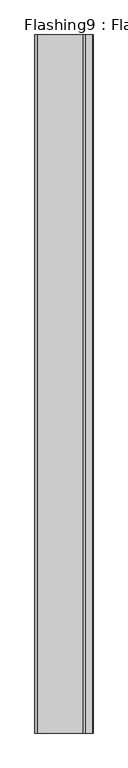
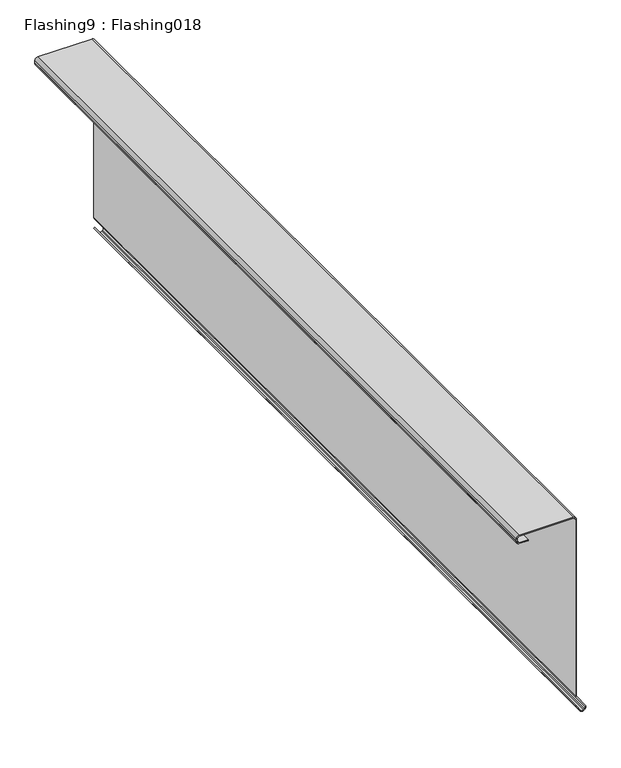
"""IFC4 building model written with IfcOpenShell, lengths in millimetres: proxy geometry, Flashing9 : Flashing018."""

import ifcopenshell
import ifcopenshell.guid

model = None  # the IFC model being written
_history = None  # IfcOwnerHistory: only IFC2X3 demands one
_inside = {}  # id of a spatial element -> (the spatial element, [elements in it])
_under = {}  # id of a project, library or spatial element -> (it, [spatial elements below it])
_declared = {}  # id of a project -> (the project, [libraries it declares])
_typed = {}  # id of a type object -> (the type object, [elements of that type])
_made_of = {}  # id of a material, layer set ... -> (it, [elements and type objects made of it])


def new_model(schema):
    """Start an empty IFC model of exactly this schema.

    Asked for "IFC4X3", IfcOpenShell would pick the latest addendum, in which some entities
    have other attributes; the version numbers below select the first issue.
    IFC2X3 requires an IfcOwnerHistory on every rooted entity: one is made here for all.
    """
    global model, _history
    if schema == "IFC4X3":
        model = ifcopenshell.file(schema_version=(4, 3, 0, 0))
    else:
        model = ifcopenshell.file(schema=schema)
    _inside.clear()
    _under.clear()
    _declared.clear()
    _typed.clear()
    _made_of.clear()
    _history = None
    if model.schema == "IFC2X3":
        org = make("IfcOrganization", Name="unknown")
        user = make(
            "IfcPersonAndOrganization",
            ThePerson=make("IfcPerson", FamilyName="unknown"),
            TheOrganization=org,
        )
        app = make(
            "IfcApplication",
            ApplicationDeveloper=org,
            Version="unknown",
            ApplicationFullName="unknown",
            ApplicationIdentifier="unknown",
        )
        _history = make(
            "IfcOwnerHistory",
            OwningUser=user,
            OwningApplication=app,
            ChangeAction="ADDED",
            CreationDate=0,
        )
    return model


def make(cls, **values):
    """One entity of the class cls with the attributes given. An attribute that is None is left unset."""
    return model.create_entity(
        cls, **{name: value for name, value in values.items() if value is not None}
    )


def rooted(cls, **values):
    """An entity with a GlobalId (a new one), such as an element, a storey or a relation."""
    return make(cls, GlobalId=ifcopenshell.guid.new(), OwnerHistory=_history, **values)


def si_unit(unit_type, name, prefix=None):
    """IfcSIUnit, for example si_unit("LENGTHUNIT", "METRE", prefix="MILLI")."""
    return make("IfcSIUnit", UnitType=unit_type, Prefix=prefix, Name=name)


def assignment(units):
    """IfcUnitAssignment: the units of a project."""
    return None if units is None else make("IfcUnitAssignment", Units=units)


def point(xyz):
    """IfcCartesianPoint."""
    return None if xyz is None else make("IfcCartesianPoint", Coordinates=xyz)


def direction(xyz):
    """IfcDirection."""
    return None if xyz is None else make("IfcDirection", DirectionRatios=xyz)


def frame(location, z_axis=None, x_axis=None):
    """IfcAxis2Placement3D, a coordinate frame: its origin and axes. An axis left out is left unset."""
    return make(
        "IfcAxis2Placement3D",
        Location=point(location),
        Axis=direction(z_axis),
        RefDirection=direction(x_axis),
    )


def frame_2d(location, x_axis=None):
    """IfcAxis2Placement2D, a coordinate frame in the plane: its origin and x axis."""
    return make(
        "IfcAxis2Placement2D", Location=point(location), RefDirection=direction(x_axis)
    )


def origin():
    """The frame at (0, 0, 0) with its axes left unset."""
    return frame((0.0, 0.0, 0.0))


def place(relative_to, where):
    """IfcLocalPlacement: puts the frame where relative to a parent placement (None: the world)."""
    return make(
        "IfcLocalPlacement", PlacementRelTo=relative_to, RelativePlacement=where
    )


def context(
    kind, dimensions, precision=None, world=None, true_north=None, identifier=None
):
    """IfcGeometricRepresentationContext, for example the 3D "Model" context."""
    return make(
        "IfcGeometricRepresentationContext",
        ContextIdentifier=identifier,
        ContextType=kind,
        CoordinateSpaceDimension=dimensions,
        Precision=precision,
        WorldCoordinateSystem=world,
        TrueNorth=true_north,
    )


def project(units=None, contexts=None):
    """IfcProject with its units and contexts."""
    return rooted(
        "IfcProject",
        Name="project",
        RepresentationContexts=contexts,
        UnitsInContext=assignment(units),
    )


def spatial(cls, under=None, at=None, **own):
    """A site, building, storey or space (cls), placed at a placement, below another one or the project."""
    s = rooted(cls, ObjectPlacement=at, **own)
    if under is not None:
        _under.setdefault(under.id(), (under, []))[1].append(s)
    return s


def polyline(points):
    """IfcPolyline through the points."""
    return make("IfcPolyline", Points=[point(p) for p in points])


def circle_curve(where, radius):
    """IfcCircle in the frame where."""
    return make("IfcCircle", Position=where, Radius=radius)


def trimmed(basis, trim1, trim2, sense, master):
    """IfcTrimmedCurve: the piece of a basis curve between two trims."""
    return make(
        "IfcTrimmedCurve",
        BasisCurve=basis,
        Trim1=trim1,
        Trim2=trim2,
        SenseAgreement=sense,
        MasterRepresentation=master,
    )


def segment(curve, same_sense, transition):
    """IfcCompositeCurveSegment."""
    return make(
        "IfcCompositeCurveSegment",
        Transition=transition,
        SameSense=same_sense,
        ParentCurve=curve,
    )


def composite_curve(segments, self_intersect=None):
    """IfcCompositeCurve: segments joined end to end."""
    return make("IfcCompositeCurve", Segments=segments, SelfIntersect=self_intersect)


def outline(outer, holes=None, kind="AREA"):
    """IfcArbitraryClosedProfileDef: a profile drawn as a closed curve; with holes, ...WithVoids."""
    if holes is None:
        return make("IfcArbitraryClosedProfileDef", ProfileType=kind, OuterCurve=outer)
    return make(
        "IfcArbitraryProfileDefWithVoids",
        ProfileType=kind,
        OuterCurve=outer,
        InnerCurves=holes,
    )


def extrude(swept, where, along, depth):
    """IfcExtrudedAreaSolid: the profile swept, set in the frame where, extruded along a direction by depth."""
    return make(
        "IfcExtrudedAreaSolid",
        SweptArea=swept,
        Position=where,
        ExtrudedDirection=direction(along),
        Depth=depth,
    )


def shape(context_of_items, identifier, shape_type, items):
    """IfcShapeRepresentation: the items that make up one representation, for example the "Body"."""
    return make(
        "IfcShapeRepresentation",
        ContextOfItems=context_of_items,
        RepresentationIdentifier=identifier,
        RepresentationType=shape_type,
        Items=items,
    )


def source(mapping_origin, context_of_items, identifier, shape_type, items):
    """IfcRepresentationMap: a shape defined once, which mapped items show again and again."""
    return make(
        "IfcRepresentationMap",
        MappingOrigin=mapping_origin,
        MappedRepresentation=shape(context_of_items, identifier, shape_type, items),
    )


def transform(
    local_origin,
    x_axis=None,
    y_axis=None,
    z_axis=None,
    scale=None,
    scale2=None,
    scale3=None,
    uniform=True,
):
    """IfcCartesianTransformationOperator3D, or its non-uniform kind. x_axis, y_axis, z_axis: its Axis1, 2, 3."""
    if uniform:
        return make(
            "IfcCartesianTransformationOperator3D",
            Axis1=direction(x_axis),
            Axis2=direction(y_axis),
            LocalOrigin=point(local_origin),
            Scale=scale,
            Axis3=direction(z_axis),
        )
    return make(
        "IfcCartesianTransformationOperator3DnonUniform",
        Axis1=direction(x_axis),
        Axis2=direction(y_axis),
        LocalOrigin=point(local_origin),
        Scale=scale,
        Axis3=direction(z_axis),
        Scale2=scale2,
        Scale3=scale3,
    )


def mapped(mapping_source, mapping_target):
    """IfcMappedItem: shows the shape of a source again, moved by a transform."""
    return make(
        "IfcMappedItem", MappingSource=mapping_source, MappingTarget=mapping_target
    )


def made_of(thing, what):
    """Note that an element or type object is made of a material, layer set ...; save() writes the relation."""
    if what is not None:
        _made_of.setdefault(what.id(), (what, []))[1].append(thing)
    return thing


def element(
    cls,
    number,
    at=None,
    inside=None,
    cuts=None,
    type_object=None,
    material=None,
    context=None,
    identifier="Body",
    shape_type=None,
    held_by="IfcProductDefinitionShape",
    body=None,
    shapes=None,
    **own,
):
    """One element of the class cls, such as IfcWall. Its Tag is "e" and its number.

    at: its placement. inside: the storey or other place that contains it. cuts: it is an
    opening in that element (IfcRelVoidsElement). A single representation is given by context,
    identifier, shape_type and body (its items); several are given by shapes. held_by: the class
    of the entity that holds the representations. save() writes the other relations.
    """
    e = rooted(cls, Tag="e%d" % number, ObjectPlacement=at, **own)
    if body is not None:
        shapes = [shape(context, identifier, shape_type, body)]
    if shapes is not None:
        e.Representation = make(held_by, Representations=shapes)
    if inside is not None:
        _inside.setdefault(inside.id(), (inside, []))[1].append(e)
    if cuts is not None:
        rooted(
            "IfcRelVoidsElement", RelatingBuildingElement=cuts, RelatedOpeningElement=e
        )
    if type_object is not None:
        _typed.setdefault(type_object.id(), (type_object, []))[1].append(e)
    return made_of(e, material)


def aggregate(whole, parts):
    """IfcRelAggregates: a whole, such as a stair, and the parts it consists of."""
    return rooted("IfcRelAggregates", RelatingObject=whole, RelatedObjects=parts)


def save(model, path):
    """Write the relations noted so far, then the file.

    IfcRelAggregates (storeys below a building ...), IfcRelContainedInSpatialStructure (elements
    in a storey), IfcRelDefinesByType, IfcRelAssociatesMaterial and IfcRelDeclares: one each for
    every whole, place, type object, material and project.
    """
    for whole, parts in _under.values():
        aggregate(whole, parts)
    for where, things in _inside.values():
        rooted(
            "IfcRelContainedInSpatialStructure",
            RelatedElements=things,
            RelatingStructure=where,
        )
    for kind, things in _typed.values():
        rooted("IfcRelDefinesByType", RelatedObjects=things, RelatingType=kind)
    for what, things in _made_of.values():
        rooted("IfcRelAssociatesMaterial", RelatedObjects=things, RelatingMaterial=what)
    for by, libraries in _declared.values():
        rooted("IfcRelDeclares", RelatingContext=by, RelatedDefinitions=libraries)
    model.write(path)


def flashing9_flashing018_9543aaf0(model_context):
    return source(origin(), model_context, "Body", "SweptSolid", [
        extrude(outline(composite_curve([segment(polyline([(43036.8907248, 17759.2743151), (43051.477598, 17749.0170677), (43050.3271805, 17747.3810543), (43035.7403074, 17757.6383018)]), True, "CONTINUOUS"), segment(trimmed(circle_curve(frame_2d((43039.8127852, 17763.429789)), 7.08), [point((43035.7403074, 17757.6383018))], [point((43034.0825771, 17767.5880476))], False, "CARTESIAN"), True, "CONTINUOUS"), segment(polyline([(43034.0825771, 17767.5880476), (43035.3752562, 17769.3693991)]), True, "CONTINUOUS"), segment(trimmed(circle_curve(frame_2d((43041.1054643, 17765.2111405)), 7.08), [point((43035.3752562, 17769.3693991))], [point((43045.1570771, 17771.0172436))], False, "CARTESIAN"), True, "CONTINUOUS"), segment(polyline([(43045.1570771, 17771.0172436), (43075.4099277, 17749.9062098)]), True, "CONTINUOUS"), segment(trimmed(circle_curve(frame_2d((43077.1724938, 17752.4320286)), 3.08), [point((43075.4099277, 17749.9062098))], [point((43077.1724938, 17749.3520286))], True, "CARTESIAN"), True, "CONTINUOUS"), segment(polyline([(43077.1724938, 17749.3520286), (43524.4015043, 17749.3520286)]), True, "CONTINUOUS"), segment(trimmed(circle_curve(frame_2d((43524.4015043, 17742.2720286)), 7.08), [point((43524.4015043, 17749.3520286))], [point((43531.4815043, 17742.2720286))], False, "CARTESIAN"), True, "CONTINUOUS"), segment(polyline([(43531.4815043, 17742.2720286), (43531.4815043, 17612.9320286)]), True, "CONTINUOUS"), segment(trimmed(circle_curve(frame_2d((43524.4015043, 17612.9320286)), 7.08), [point((43531.4815043, 17612.9320286))], [point((43524.4015043, 17605.8520286))], False, "CARTESIAN"), True, "CONTINUOUS"), segment(polyline([(43524.4015043, 17605.8520286), (43517.995098, 17605.8520286)]), True, "CONTINUOUS"), segment(trimmed(circle_curve(frame_2d((43517.995098, 17612.9320286)), 7.08), [point((43517.995098, 17605.8520286))], [point((43510.915098, 17612.9320286))], False, "CARTESIAN"), True, "CONTINUOUS"), segment(polyline([(43510.915098, 17612.9320286), (43510.915098, 17634.2284935), (43512.915098, 17634.2284935), (43512.915098, 17612.9320286)]), True, "CONTINUOUS"), segment(trimmed(circle_curve(frame_2d((43517.995098, 17612.9320286)), 5.08), [point((43512.915098, 17612.9320286))], [point((43517.995098, 17607.8520286))], True, "CARTESIAN"), True, "CONTINUOUS"), segment(polyline([(43517.995098, 17607.8520286), (43524.4015043, 17607.8520286)]), True, "CONTINUOUS"), segment(trimmed(circle_curve(frame_2d((43524.4015043, 17612.9320286)), 5.08), [point((43524.4015043, 17607.8520286))], [point((43529.4815043, 17612.9320286))], True, "CARTESIAN"), True, "CONTINUOUS"), segment(polyline([(43529.4815043, 17612.9320286), (43529.4815043, 17742.2720286)]), True, "CONTINUOUS"), segment(trimmed(circle_curve(frame_2d((43524.4015043, 17742.2720286)), 5.08), [point((43529.4815043, 17742.2720286))], [point((43524.4015043, 17747.3520286))], True, "CARTESIAN"), True, "CONTINUOUS"), segment(polyline([(43524.4015043, 17747.3520286), (43077.1724938, 17747.3520286)]), True, "CONTINUOUS"), segment(trimmed(circle_curve(frame_2d((43077.1724938, 17752.4320286)), 5.08), [point((43077.1724938, 17747.3520286))], [point((43074.2654043, 17748.2660676))], False, "CARTESIAN"), True, "CONTINUOUS"), segment(polyline([(43074.2654043, 17748.2660676), (43044.0125537, 17769.3771014)]), True, "CONTINUOUS"), segment(trimmed(circle_curve(frame_2d((43041.1054643, 17765.2111405)), 5.08), [point((43044.0125537, 17769.3771014))], [point((43036.993959, 17768.1947498))], True, "CARTESIAN"), True, "CONTINUOUS"), segment(polyline([(43036.993959, 17768.1947498), (43035.7012799, 17766.4133983)]), True, "CONTINUOUS"), segment(trimmed(circle_curve(frame_2d((43039.8127852, 17763.429789)), 5.08), [point((43035.7012799, 17766.4133983))], [point((43036.8907248, 17759.2743151))], True, "CARTESIAN"), True, "CONTINUOUS")], self_intersect=False)), frame((0.0, 7982.1507711, 0.0), z_axis=(0.0, 1.0, 0.0), x_axis=(0.0, 0.0, 1.0)), (0.0, 0.0, 1.0), 2000.0),
    ])


if __name__ == "__main__":
    model = new_model("IFC4")
    model_context = context("Model", 3, world=origin())
    ifc_project = project(units=[si_unit("LENGTHUNIT", "METRE", prefix="MILLI")], contexts=[model_context])
    site = spatial("IfcSite", under=ifc_project)
    building = spatial("IfcBuilding", under=site)
    placement = place(None, origin())
    flashing9_flashing018_shape = flashing9_flashing018_9543aaf0(model_context)
    element("IfcBuildingElementProxy", 1, Name="Flashing9 : Flashing018", ObjectType="Flashing9 : Flashing018", at=placement, inside=building, context=model_context, shape_type="MappedRepresentation", body=[
        mapped(flashing9_flashing018_shape, transform((0.0, 0.0, 0.0), x_axis=(1.0, 0.0, 0.0), y_axis=(0.0, 1.0, 0.0), z_axis=(0.0, 0.0, 1.0))),
    ])
    save(model, "model.ifc")

# Revit data of these elements
# Type "Flashing9 : Flashing018"
#   NameOverride = "Flashing018"
# Element 1 (IfcBuildingElementProxy, "Flashing9 : Flashing018")
#   Materials on its faces: "HIGH EAVE FLASHING"
# Materials
#   "HIGH EAVE FLASHING": class "Unassigned", colour RGB 128 128 128, transparency 0, Cost = 0
